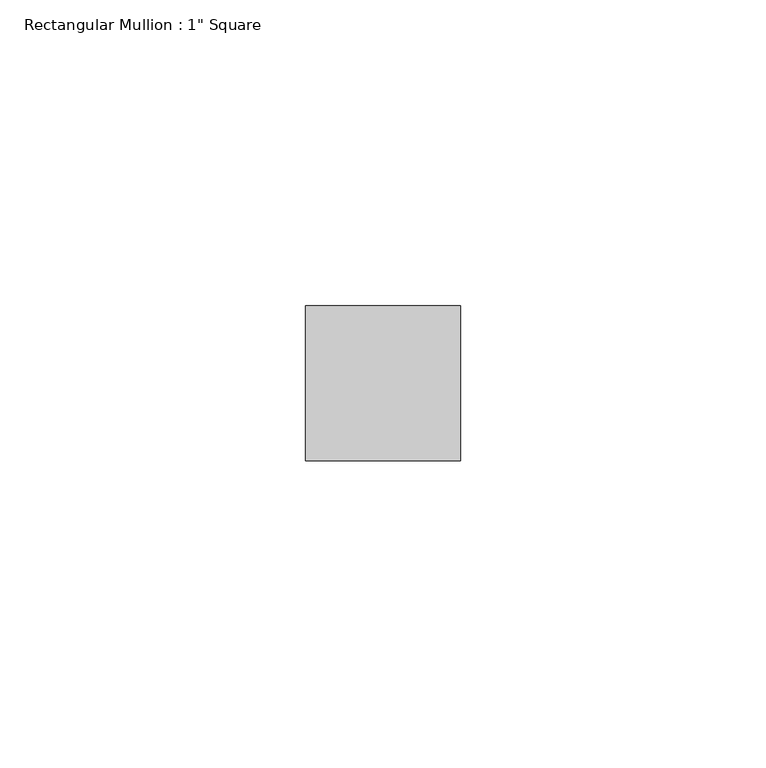
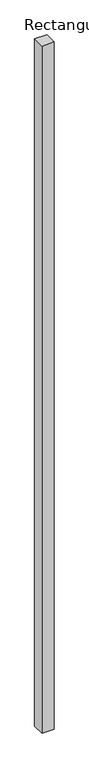
"""IFC4 building model written with IfcOpenShell, lengths in millimetres: member geometry."""

from ifc_helpers import new_model, si_unit, frame, origin, place, context, project, spatial, polyline, outline, extrude, source, transform, mapped, element, save


def member_31180177(model_context):
    return source(origin(), model_context, "Body", "SweptSolid", [
        extrude(outline(polyline([(0.0, 12.7), (0.0, -12.7), (-25.4, -12.7), (-25.4, 12.7), (0.0, 12.7)])), frame((0.0, 0.0, -1498.6000003), z_axis=(0.0, 0.0, 1.0), x_axis=(1.0, 0.0, 0.0)), (0.0, 0.0, 1.0), 1498.6000003),
    ])


if __name__ == "__main__":
    model = new_model("IFC4")
    model_context = context("Model", 3, world=origin())
    ifc_project = project(units=[si_unit("LENGTHUNIT", "METRE", prefix="MILLI")], contexts=[model_context])
    site = spatial("IfcSite", under=ifc_project)
    building = spatial("IfcBuilding", under=site)
    placement = place(None, origin())
    member_shape = member_31180177(model_context)
    element("IfcMember", 1, ObjectType="Rectangular Mullion : 1\" Square", at=placement, inside=building, context=model_context, shape_type="MappedRepresentation", body=[
        mapped(member_shape, transform((0.0, 0.0, 0.0), x_axis=(1.0, 0.0, 0.0), y_axis=(0.0, 1.0, 0.0), z_axis=(0.0, 0.0, 1.0))),
    ])
    save(model, "model.ifc")

# Revit data of these elements
# Type "Rectangular Mullion : 1\" Square"
#   built-in parameter 1007304 = 0.0833333 (stored number, unit not read)
#   built-in parameter 1007301 = 0.0416667 (stored number, unit not read)
#   built-in parameter 1007300 = 0.0416667 (stored number, unit not read)
# Element 1 (IfcMember, "Rectangular Mullion : 1\" Square")
#   Materials on its faces: "Metal - Aluminum"
# Materials
#   "Metal - Aluminum": class "Metal", colour RGB 247 247 247, transparency 0
